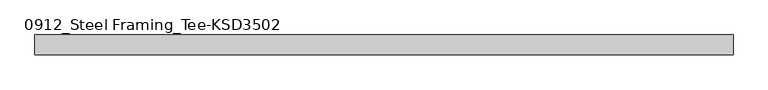
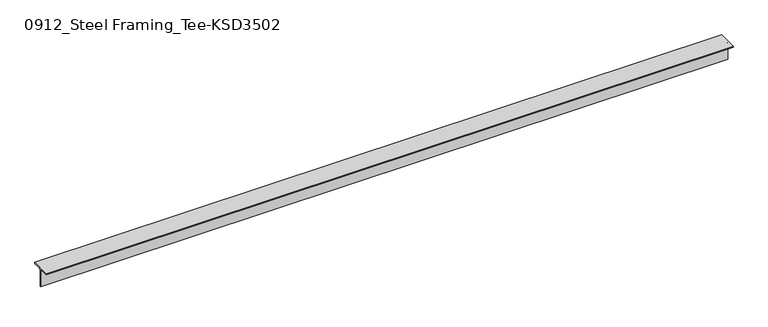
"""IFC4 building model written with IfcOpenShell, lengths in millimetres: member geometry, 0912_Steel Framing_Tee-KSD3502 : H_SB_ASB_CT-150x150x6.5x9."""

from ifc_helpers import new_model, si_unit, point, frame, frame_2d, origin, place, context, project, spatial, polyline, circle_curve, trimmed, segment, composite_curve, outline, extrude, source, transform, mapped, element, save


def member_0912_steel_framing_tee_ksd3502_6fd16e1c(model_context):
    return source(origin(), model_context, "Body", "SweptSolid", [
        extrude(outline(composite_curve([segment(polyline([(-75.0, 75.0), (75.0, 75.0), (75.0, 66.0), (16.25, 66.0)]), True, "CONTINUOUS"), segment(trimmed(circle_curve(frame_2d((16.25, 53.0)), 13.0), [point((16.25, 66.0))], [point((3.25, 53.0))], True, "CARTESIAN"), True, "CONTINUOUS"), segment(polyline([(3.25, 53.0), (3.25, -75.0), (-3.25, -75.0), (-3.25, 53.0)]), True, "CONTINUOUS"), segment(trimmed(circle_curve(frame_2d((-16.25, 53.0)), 13.0), [point((-3.25, 53.0))], [point((-16.25, 66.0))], True, "CARTESIAN"), True, "CONTINUOUS"), segment(polyline([(-16.25, 66.0), (-75.0, 66.0), (-75.0, 75.0)]), True, "CONTINUOUS")], self_intersect=False)), frame((-2577.05, 0.0, 0.0), z_axis=(1.0, 0.0, 0.0), x_axis=(0.0, 1.0, 0.0)), (0.0, 0.0, 1.0), 5312.4),
    ])


if __name__ == "__main__":
    model = new_model("IFC4")
    model_context = context("Model", 3, world=origin())
    ifc_project = project(units=[si_unit("LENGTHUNIT", "METRE", prefix="MILLI")], contexts=[model_context])
    site = spatial("IfcSite", under=ifc_project)
    building = spatial("IfcBuilding", under=site)
    placement = place(None, origin())
    member_0912_steel_framing_tee_ksd3502_shape = member_0912_steel_framing_tee_ksd3502_6fd16e1c(model_context)
    element("IfcMember", 1, ObjectType="0912_Steel Framing_Tee-KSD3502 : H_SB_ASB_CT-150x150x6.5x9", at=placement, inside=building, context=model_context, shape_type="MappedRepresentation", body=[
        mapped(member_0912_steel_framing_tee_ksd3502_shape, transform((0.0, 0.0, 0.0), x_axis=(1.0, 0.0, 0.0), y_axis=(0.0, 1.0, 0.0), z_axis=(0.0, 0.0, 1.0))),
    ])
    save(model, "model.ifc")

# Revit data of these elements
# Type "0912_Steel Framing_Tee-KSD3502 : H_SB_ASB_CT-150x150x6.5x9"
#   H_WM Code_1 = "S01AA003-00001 | Main Steel Structure Fabrication Work | Shelter/Building | Light Steel - Standard (30KG/M>Weight) | Material: (   )"
#   H_WM Code_2 = "S03AA029-00001 | Main Steel Structure Erection Work | Shelter/Building | Light Steel (30KG/M>Weight) | Material: (   )"
#   H_WM Code_3 = "S01AA010-00001 | Main Steel Structure Fabrication Work | Shelter/Building | Steel Painting/Coating | for Non-Fireproofed Steel Surface, Surface Preparation, Primer, Second & Final Coat | Material: (   )"
#   H_Q'ty Cal Type Tag = "SB-Q2"
#   Width = 15.0 cm
#   Web Thickness = 0.65 cm
#   Web Fillet = 1.3 cm
#   Section Area = 23.39 cm²
#   Perimeter = 0.60 m²/m
#   Nominal Weight = 18.40 kgf/m
#   Height = 15.0 cm
#   Flange Thickness = 0.9 cm
#   Centroid Vertical = 7.5 cm
#   Centroid Horizontal = 7.5 cm
#   Length [instance default] = 1.5000 m
#   Structural Material [instance default] = Steel, 45-345
#   Warping Constant = (empty or 0)
#   Torsional Moment of Inertia = 0
#   Section Name Key = ""
#   Plastic Modulus weak axis = 0
#   Plastic Modulus strong axis = 0
#   Moment of Inertia weak axis = 0
#   Moment of Inertia strong axis = 0
#   Elastic Modulus weak axis = 0
#   Elastic Modulus strong axis = 0
#   Bolt Spacing = 0
#   Assembly Code = ""
# Element 1 (IfcMember, "0912_Steel Framing_Tee-KSD3502 : H_SB_ASB_CT-150x150x6.5x9")
#   Structural Material = none
# Materials
#   "Steel, 45-345": class "Metal", colour RGB 189 187 185, transparency 0, Description = "Steel 345 MPa", Cost = 0
